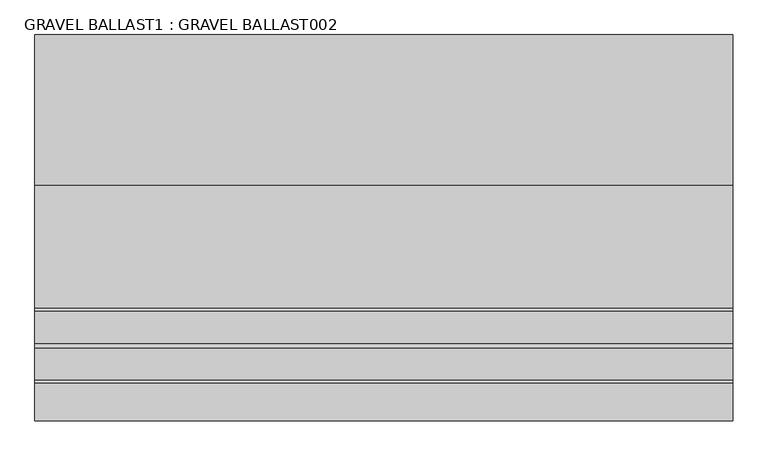
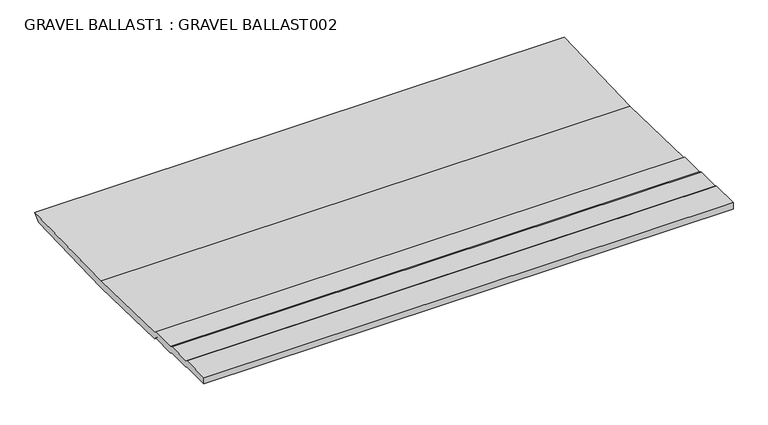
"""IFC4 building model written with IfcOpenShell, lengths in millimetres: proxy geometry, GRAVEL BALLAST1 : GRAVEL BALLAST002."""

from ifc_helpers import new_model, si_unit, frame, origin, place, context, project, spatial, polyline, outline, extrude, source, transform, mapped, element, save


def gravel_ballast1_gravel_ballast002_c19f6b3d(model_context):
    return source(origin(), model_context, "Body", "SweptSolid", [
        extrude(outline(polyline([(-5440.365918, 40253.79375), (-5549.8654297, 40253.79375), (-5549.8654297, 40278.5320313), (-5440.365918, 40278.5320313), (-5431.6554687, 40274.2507813), (-5341.0685547, 40274.2507813), (-5328.2239153, 40268.5233193), (-5234.272168, 40270.16875), (-5225.9987305, 40262.7585938), (-4873.4420898, 40254.5398438), (-4442.8393555, 40268.1982422), (-4468.0649414, 40242.9726562), (-4873.4420898, 40229.8015625), (-5225.9987305, 40238.0203125), (-5234.272168, 40245.4304687), (-5328.2239153, 40243.785038), (-5341.0685547, 40249.5125), (-5431.6554687, 40249.5125), (-5440.365918, 40253.79375)])), frame((12382.7678845, 0.0, 0.0), z_axis=(1.0, 0.0, 0.0), x_axis=(0.0, 1.0, 0.0)), (0.0, 0.0, 1.0), 2000.0),
    ])


if __name__ == "__main__":
    model = new_model("IFC4")
    model_context = context("Model", 3, world=origin())
    ifc_project = project(units=[si_unit("LENGTHUNIT", "METRE", prefix="MILLI")], contexts=[model_context])
    site = spatial("IfcSite", under=ifc_project)
    building = spatial("IfcBuilding", under=site)
    placement = place(None, origin())
    gravel_ballast1_gravel_ballast002_shape = gravel_ballast1_gravel_ballast002_c19f6b3d(model_context)
    element("IfcBuildingElementProxy", 1, Name="GRAVEL BALLAST1 : GRAVEL BALLAST002", ObjectType="GRAVEL BALLAST1 : GRAVEL BALLAST002", at=placement, inside=building, context=model_context, shape_type="MappedRepresentation", body=[
        mapped(gravel_ballast1_gravel_ballast002_shape, transform((0.0, 0.0, 0.0), x_axis=(1.0, 0.0, 0.0), y_axis=(0.0, 1.0, 0.0), z_axis=(0.0, 0.0, 1.0))),
    ])
    save(model, "model.ifc")

# Revit data of these elements
# Type "GRAVEL BALLAST1 : GRAVEL BALLAST002"
#   NameOverride = "GRAVEL BALLAST002"
# Element 1 (IfcBuildingElementProxy, "GRAVEL BALLAST1 : GRAVEL BALLAST002")
#   Materials on its faces: "GRAVEL BALLAST"
# Materials
#   "GRAVEL BALLAST": class "Unassigned", colour RGB 128 128 128, transparency 0, Cost = 0
